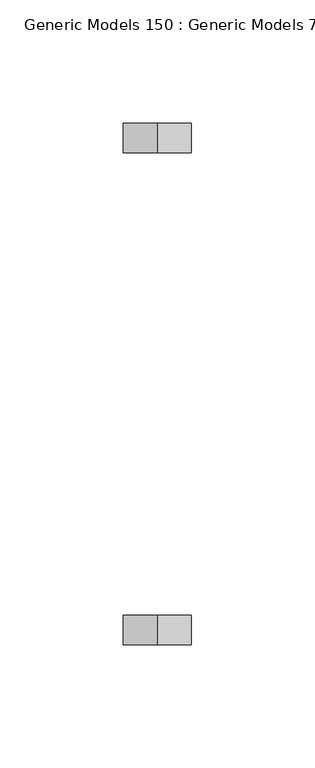
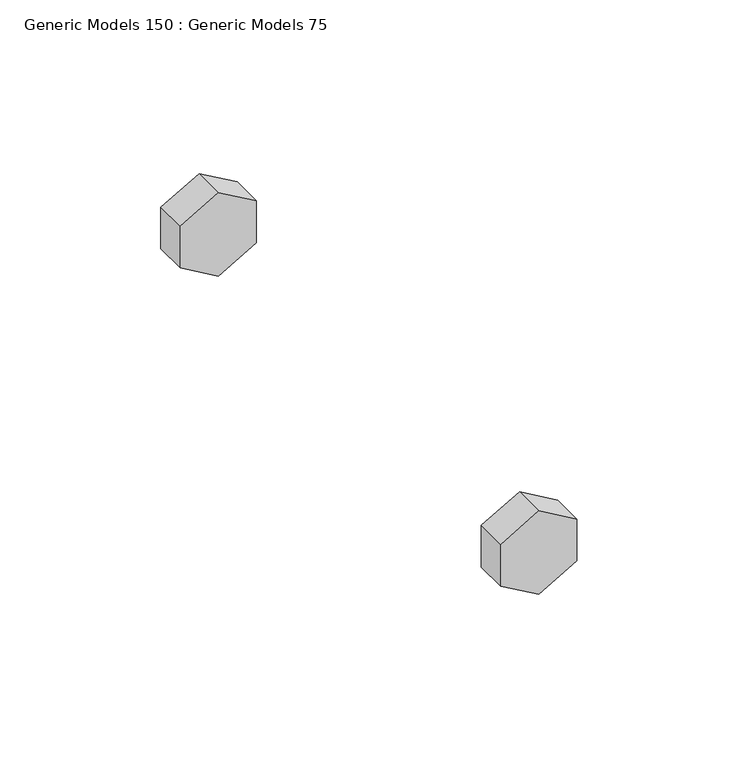
"""IFC4 building model written with IfcOpenShell, lengths in millimetres: proxy geometry, Generic Models 150 : Generic Models 75."""

from ifc_helpers import new_model, si_unit, frame, origin, place, context, project, spatial, polyline, outline, extrude, source, transform, mapped, element, save


def generic_models_150_generic_models_75_63bd89ca(model_context):
    return source(origin(), model_context, "Body", "SweptSolid", [
        extrude(outline(polyline([(268993.7462802, 31975.9942029), (268977.9097067, 31975.9942029), (268969.99142, 31989.7090778), (268977.9097067, 32003.4239528), (268993.7462802, 32003.4239528), (269001.664567, 31989.7090778), (268993.7462802, 31975.9942029)])), frame((0.0, 30868.0031612, 0.0), z_axis=(0.0, 1.0, 0.0), x_axis=(0.0, 0.0, 1.0)), (0.0, 0.0, 1.0), 11.90625),
        extrude(outline(polyline([(268993.7462802, 31975.9942029), (268977.9097067, 31975.9942029), (268969.99142, 31989.7090778), (268977.9097067, 32003.4239528), (268993.7462802, 32003.4239528), (269001.664567, 31989.7090778), (268993.7462802, 31975.9942029)])), frame((0.0, 30668.7719112, 0.0), z_axis=(0.0, 1.0, 0.0), x_axis=(0.0, 0.0, 1.0)), (0.0, 0.0, 1.0), 11.90625),
    ])


if __name__ == "__main__":
    model = new_model("IFC4")
    model_context = context("Model", 3, world=origin())
    ifc_project = project(units=[si_unit("LENGTHUNIT", "METRE", prefix="MILLI")], contexts=[model_context])
    site = spatial("IfcSite", under=ifc_project)
    building = spatial("IfcBuilding", under=site)
    placement = place(None, origin())
    generic_models_150_generic_models_75_shape = generic_models_150_generic_models_75_63bd89ca(model_context)
    element("IfcBuildingElementProxy", 1, Name="Generic Models 150 : Generic Models 75", ObjectType="Generic Models 150 : Generic Models 75", at=placement, inside=building, context=model_context, shape_type="MappedRepresentation", body=[
        mapped(generic_models_150_generic_models_75_shape, transform((0.0, 0.0, 0.0), x_axis=(1.0, 0.0, 0.0), y_axis=(0.0, 1.0, 0.0), z_axis=(0.0, 0.0, 1.0))),
    ])
    save(model, "model.ifc")

# Revit data of these elements
# Element 1 (IfcBuildingElementProxy, "Generic Models 150 : Generic Models 75")
#   Materials on its faces: "3/4\" GALV. THRU BOLTS"
# Materials
#   "3/4\" GALV. THRU BOLTS": class "Generic", colour RGB 105 69 171, transparency 0, Cost = 0
